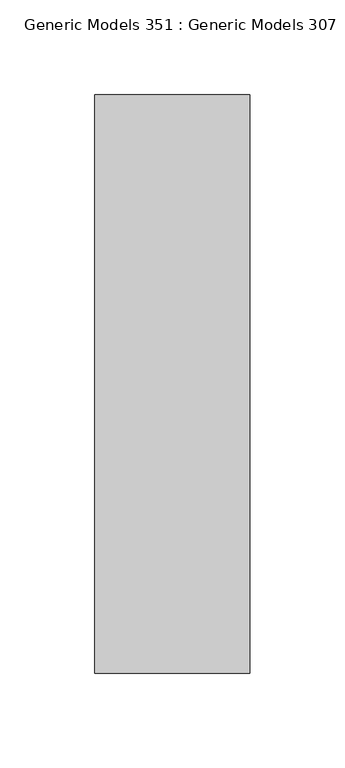
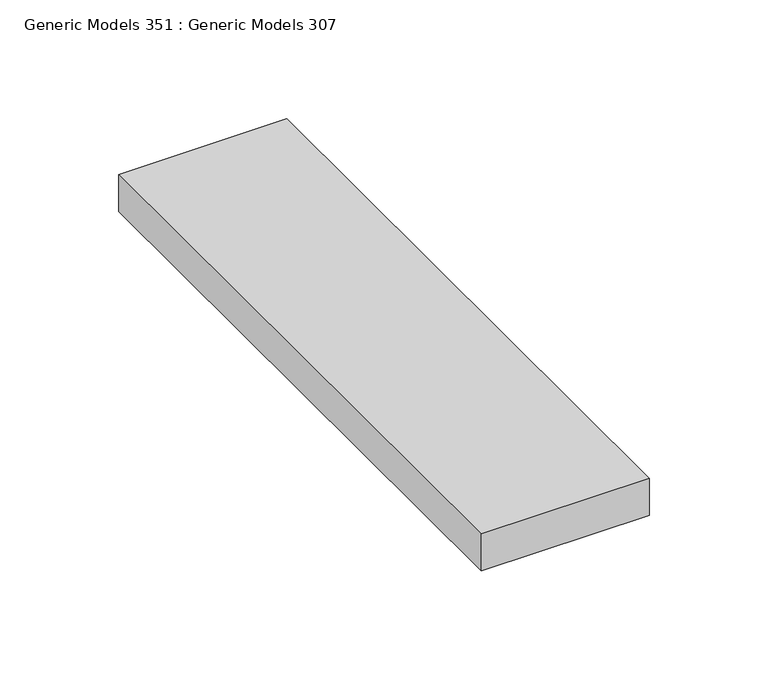
"""IFC4 building model written with IfcOpenShell, lengths in millimetres: proxy geometry, Generic Models 351 : Generic Models 307."""

from ifc_helpers import new_model, si_unit, frame, origin, place, context, project, spatial, polyline, outline, extrude, source, transform, mapped, element, save


def generic_models_351_generic_models_307_6b136326(model_context):
    return source(origin(), model_context, "Body", "SweptSolid", [
        extrude(outline(polyline([(4839.3786898, 704.5309662), (4921.0763704, 704.5309662), (4921.0763704, 399.7309662), (4839.3786898, 399.7309662), (4839.3786898, 704.5309662)])), frame((0.0, 0.0, 129228.596), z_axis=(0.0, 0.0, 1.0), x_axis=(1.0, 0.0, 0.0)), (0.0, 0.0, 1.0), 19.05),
    ])


if __name__ == "__main__":
    model = new_model("IFC4")
    model_context = context("Model", 3, world=origin())
    ifc_project = project(units=[si_unit("LENGTHUNIT", "METRE", prefix="MILLI")], contexts=[model_context])
    site = spatial("IfcSite", under=ifc_project)
    building = spatial("IfcBuilding", under=site)
    placement = place(None, origin())
    generic_models_351_generic_models_307_shape = generic_models_351_generic_models_307_6b136326(model_context)
    element("IfcBuildingElementProxy", 1, Name="Generic Models 351 : Generic Models 307", ObjectType="Generic Models 351 : Generic Models 307", at=placement, inside=building, context=model_context, shape_type="MappedRepresentation", body=[
        mapped(generic_models_351_generic_models_307_shape, transform((0.0, 0.0, 0.0), x_axis=(1.0, 0.0, 0.0), y_axis=(0.0, 1.0, 0.0), z_axis=(0.0, 0.0, 1.0))),
    ])
    save(model, "model.ifc")

# Revit data of these elements
# Element 1 (IfcBuildingElementProxy, "Generic Models 351 : Generic Models 307")
#   Materials on its faces: "_BLOCKING AS REQUIRED"
# Materials
#   "_BLOCKING AS REQUIRED": class "Generic", colour RGB 177 130 114, transparency 0, Cost = 0
